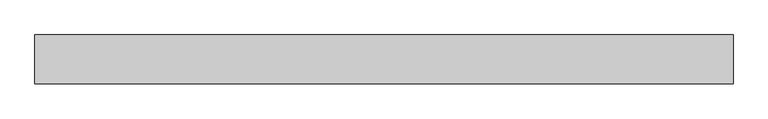
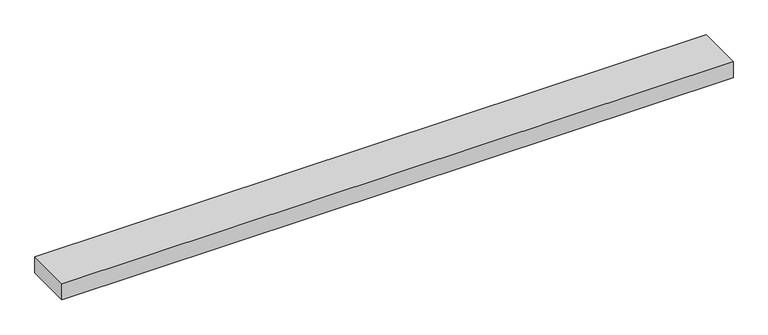
"""IFC4 building model written with IfcOpenShell, lengths in millimetres: proxy geometry, Blocking014 3031 : Blocking014 3031."""

from ifc_helpers import new_model, si_unit, frame, origin, place, context, project, spatial, polyline, outline, extrude, source, transform, mapped, element, save


def generic_models_2ca3b9cd(model_context):
    return source(origin(), model_context, "Body", "SweptSolid", [
        extrude(outline(polyline([(3694.2883192, 10278.0250834), (3694.2883192, 10417.7250834), (5694.2883192, 10417.7250834), (5694.2883192, 10278.0250834), (3694.2883192, 10278.0250834)])), frame((0.0, 0.0, 43277.559375), z_axis=(0.0, 0.0, 1.0), x_axis=(1.0, 0.0, 0.0)), (0.0, 0.0, 1.0), 50.8),
    ])


if __name__ == "__main__":
    model = new_model("IFC4")
    model_context = context("Model", 3, world=origin())
    ifc_project = project(units=[si_unit("LENGTHUNIT", "METRE", prefix="MILLI")], contexts=[model_context])
    site = spatial("IfcSite", under=ifc_project)
    building = spatial("IfcBuilding", under=site)
    placement = place(None, origin())
    generic_models_shape = generic_models_2ca3b9cd(model_context)
    element("IfcBuildingElementProxy", 1, Name="Blocking014 3031 : Blocking014 3031", ObjectType="Blocking014 3031 : Blocking014 3031", at=placement, inside=building, context=model_context, shape_type="MappedRepresentation", body=[
        mapped(generic_models_shape, transform((0.0, 0.0, 0.0), x_axis=(1.0, 0.0, 0.0), y_axis=(0.0, 1.0, 0.0), z_axis=(0.0, 0.0, 1.0))),
    ])
    save(model, "model.ifc")

# Revit data of these elements
# Type "Blocking014 3031 : Blocking014 3031"
#   NameOverride = "Blocking014"
# Element 1 (IfcBuildingElementProxy, "Blocking014 3031 : Blocking014 3031")
#   Materials on its faces: "WOOD BLOCKING AS REQUIRED"
# Materials
#   "WOOD BLOCKING AS REQUIRED": class "Unassigned", colour RGB 166 124 85, transparency 0, Cost = 0
